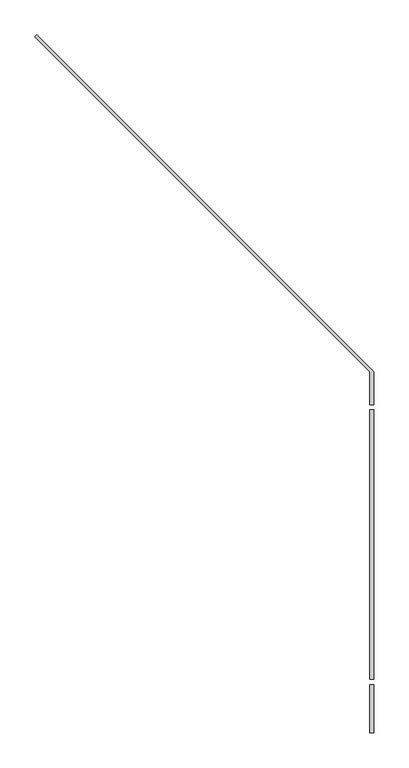
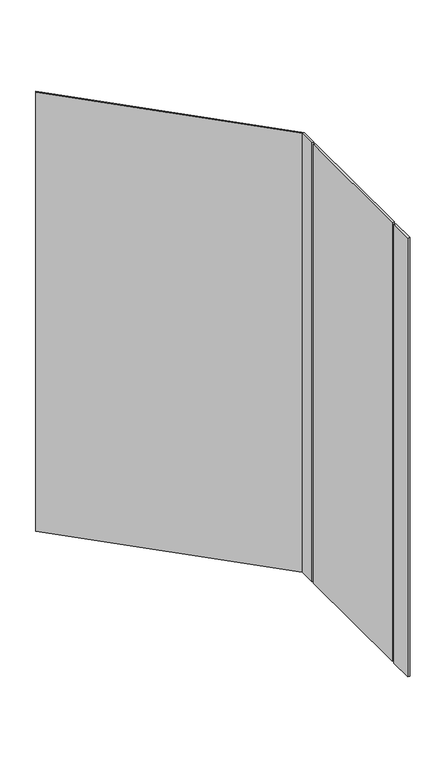
"""IFC4 building model written with IfcOpenShell, lengths in millimetres: furniture geometry, MB SHower Encloser : MB SHower Encloser."""

from ifc_helpers import new_model, si_unit, frame, origin, place, context, project, spatial, polyline, outline, extrude, source, transform, mapped, element, save


def furniture_cca0b65e(model_context):
    return source(origin(), model_context, "Body", "SweptSolid", [
        extrude(outline(polyline([(-9419.845921, 14259.304079), (-8673.3163337, 13512.7744917), (-8673.3163337, 13439.3065595), (-8682.526071, 13439.3065595), (-8682.526071, 13513.0039729), (-9424.336049, 14254.813951), (-9419.845921, 14259.304079)])), frame((0.0, 0.0, 101.6), z_axis=(0.0, 0.0, 1.0), x_axis=(1.0, 0.0, 0.0)), (0.0, 0.0, 1.0), 2032.0),
        extrude(outline(polyline([(-8673.3163337, 12712.7), (-8682.4936305, 12712.7), (-8682.4936305, 12819.2414063), (-8673.3163337, 12819.2414063), (-8673.3163337, 12712.7)])), frame((0.0, 0.0, 101.6), z_axis=(0.0, 0.0, 1.0), x_axis=(1.0, 0.0, 0.0)), (0.0, 0.0, 1.0), 2032.0),
        extrude(outline(polyline([(-8682.4936305, 12831.1346455), (-8682.4936305, 13428.6402985), (-8673.3163337, 13428.6402985), (-8673.3163337, 12831.1346455), (-8682.4936305, 12831.1346455)])), frame((0.0, 0.0, 101.6), z_axis=(0.0, 0.0, 1.0), x_axis=(1.0, 0.0, 0.0)), (0.0, 0.0, 1.0), 2032.0),
    ])


if __name__ == "__main__":
    model = new_model("IFC4")
    model_context = context("Model", 3, world=origin())
    ifc_project = project(units=[si_unit("LENGTHUNIT", "METRE", prefix="MILLI")], contexts=[model_context])
    site = spatial("IfcSite", under=ifc_project)
    building = spatial("IfcBuilding", under=site)
    placement = place(None, origin())
    furniture_shape = furniture_cca0b65e(model_context)
    element("IfcFurniture", 1, ObjectType="MB SHower Encloser : MB SHower Encloser", at=placement, inside=building, context=model_context, shape_type="MappedRepresentation", body=[
        mapped(furniture_shape, transform((0.0, 0.0, 0.0), x_axis=(1.0, 0.0, 0.0), y_axis=(0.0, 1.0, 0.0), z_axis=(0.0, 0.0, 1.0))),
    ])
    save(model, "model.ifc")

# Revit data of these elements
# Type "MB SHower Encloser : MB SHower Encloser"
#   COBie.Type = no
# Element 1 (IfcFurniture, "MB SHower Encloser : MB SHower Encloser")
#   Materials on its faces: "Glass"
# Materials
#   "Glass": class "Glass", colour RGB 0 128 192, transparency 0.75, Description = "Soda Lime Glass", Cost = 0
